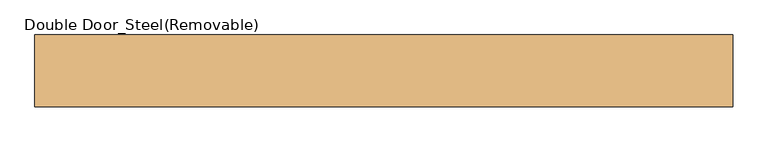
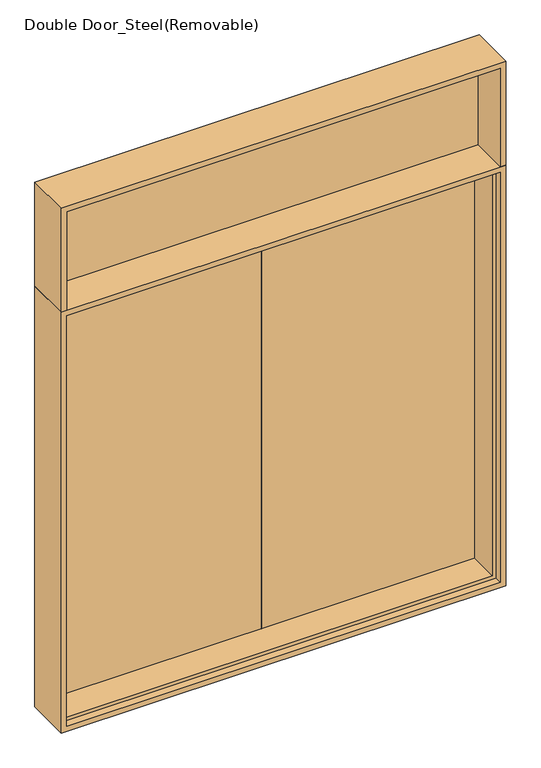
"""IFC4 building model written with IfcOpenShell, lengths in millimetres: door geometry, Double Door_Steel(Removable) : H_DR_AR B12_Door_Double_W2460xH3045_No FR_SD-7."""

from ifc_helpers import new_model, si_unit, frame, origin, place, context, project, spatial, polyline, outline, extrude, faceted_brep, source, transform, mapped, element, save


def double_door_steel_removable_5e6fc9dd(model_context):
    return source(origin(), model_context, "Body", "SolidModel", [
        faceted_brep([(-1215.0, -125.0, 2430.0), (-1215.0, 125.0, 2430.0), (-1215.0, 125.0, 0.0), (-1215.0, -125.0, 0.0), (1215.0, 125.0, 0.0), (1215.0, 125.0, 2430.0), (1185.0, 125.0, 2400.0), (-1185.0, 125.0, 2400.0), (-1185.0, 125.0, 30.0), (1185.0, 125.0, 30.0), (1215.0, -125.0, 0.0), (1215.0, -125.0, 2430.0), (1185.0, -125.0, 30.0), (-1185.0, -125.0, 30.0), (-1185.0, -125.0, 2400.0), (1185.0, -125.0, 2400.0), (-1185.0, -85.0, 2400.0), (-1185.0, -85.0, 30.0), (1185.0, -85.0, 30.0), (1185.0, -85.0, 2400.0), (1165.0, -85.0, 2380.0), (1165.0, -85.0, 50.0), (-1165.0, -85.0, 50.0), (-1165.0, -85.0, 2380.0), (-1165.0, 85.0, 2380.0), (-1165.0, 85.0, 50.0), (1165.0, 85.0, 50.0), (1185.0, 85.0, 30.0), (-1185.0, 85.0, 30.0), (-1185.0, 85.0, 2400.0), (1185.0, 85.0, 2400.0), (1165.0, 85.0, 2380.0)], [[[0, 1, 2, 3]], [[4, 2, 1, 5], [6, 7, 8, 9]], [[3, 2, 4, 10]], [[11, 0, 3, 10], [12, 13, 14, 15]], [[16, 14, 13, 17]], [[17, 13, 12, 18]], [[16, 17, 18, 19], [20, 21, 22, 23]], [[24, 23, 22, 25]], [[25, 22, 21, 26]], [[27, 28, 29, 30], [31, 24, 25, 26]], [[7, 29, 28, 8]], [[8, 28, 27, 9]], [[10, 4, 5, 11]], [[9, 27, 30, 6]], [[18, 12, 15, 19]], [[26, 21, 20, 31]], [[11, 5, 1, 0]], [[19, 15, 14, 16]], [[31, 20, 23, 24]], [[6, 30, 29, 7]]]),
        extrude(outline(polyline([(1185.0, 85.0), (0.0, 85.0), (0.0, 125.0), (1185.0, 125.0), (1185.0, 85.0)])), frame((0.0, 0.0, 30.0), z_axis=(0.0, 0.0, 1.0), x_axis=(1.0, 0.0, 0.0)), (0.0, 0.0, 1.0), 2370.0),
        extrude(outline(polyline([(0.0, 85.0), (-1185.0, 85.0), (-1185.0, 125.0), (0.0, 125.0), (0.0, 85.0)])), frame((0.0, 0.0, 30.0), z_axis=(0.0, 0.0, 1.0), x_axis=(1.0, 0.0, 0.0)), (0.0, 0.0, 1.0), 2370.0),
        extrude(outline(polyline([(1185.0, 85.0), (-1185.0, 85.0), (-1185.0, 125.0), (1185.0, 125.0), (1185.0, 85.0)])), frame((0.0, 0.0, 2430.0), z_axis=(0.0, 0.0, 1.0), x_axis=(1.0, 0.0, 0.0)), (0.0, 0.0, 1.0), 570.0),
        extrude(outline(polyline([(3030.0, 1215.0), (3030.0, -1215.0), (2430.0, -1215.0), (2430.0, -1185.0), (3000.0, -1185.0), (3000.0, 1185.0), (2430.0, 1185.0), (2430.0, 1215.0), (3030.0, 1215.0)])), frame((0.0, -125.0, 0.0), z_axis=(0.0, 1.0, 0.0), x_axis=(0.0, 0.0, 1.0)), (0.0, 0.0, 1.0), 250.0),
    ])


if __name__ == "__main__":
    model = new_model("IFC4")
    model_context = context("Model", 3, world=origin())
    ifc_project = project(units=[si_unit("LENGTHUNIT", "METRE", prefix="MILLI")], contexts=[model_context])
    site = spatial("IfcSite", under=ifc_project)
    building = spatial("IfcBuilding", under=site)
    placement = place(None, origin())
    double_door_steel_removable_shape = double_door_steel_removable_5e6fc9dd(model_context)
    element("IfcDoor", 1, ObjectType="Double Door_Steel(Removable) : H_DR_AR B12_Door_Double_W2460xH3045_No FR_SD-7", at=placement, inside=building, context=model_context, shape_type="MappedRepresentation", body=[
        mapped(double_door_steel_removable_shape, transform((0.0, 0.0, 0.0), x_axis=(1.0, 0.0, 0.0), y_axis=(0.0, 1.0, 0.0), z_axis=(0.0, 0.0, 1.0))),
    ])
    save(model, "model.ifc")

# Revit data of these elements
# Type "Double Door_Steel(Removable) : H_DR_AR B12_Door_Double_W2460xH3045_No FR_SD-7"
#   Type Mark = "464"
#   프레임 = ""
#   철물 = ""
#   유리/마감 = ""
#   위치/개소 = ""
#   부호 = ""
#   문번호 = ""
#   문기호 = "SD-7"
#   Analytic Construction = "<None>"
#   Removable Height = 600 mm
#   Door Width = 1185 mm
#   Height = 2430 mm
#   Width = 2460 mm
#   Define Thermal Properties by = 1
#   문 틀 = none
#   문 = none
#   Function = (empty or 0)
#   Assembly Code = ""
#   Wall Closure = (empty or 0)
# Element 1 (IfcDoor, "Double Door_Steel(Removable) : H_DR_AR B12_Door_Double_W2460xH3045_No FR_SD-7")
#   Materials on its faces: "00_Metal_Steel"
# Materials
#   "00_Metal_Steel": class "Metal", colour RGB 148 148 148, transparency 0, Description = "Steel", Cost = 0, Image = Doors - Windows.Glazed Curtain Walls.Stainless Steel Curtain Wall.jpg
